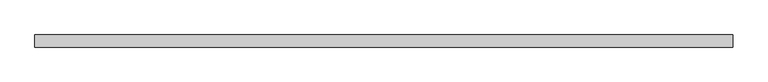
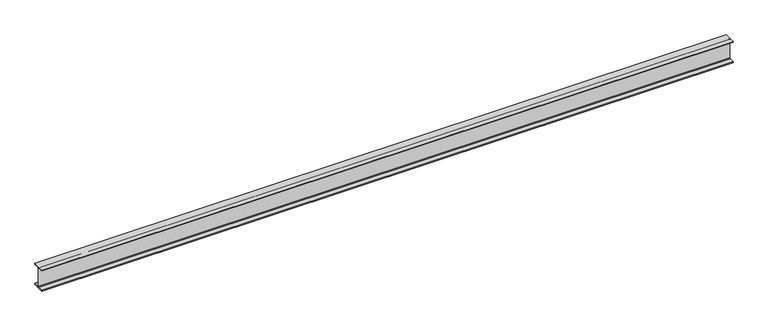
"""IFC4 building model written with IfcOpenShell, lengths in millimetres: beam geometry, Old_Steel Beam_H-KSD3502 : H_SB_ASB_H-350×175x7x11."""

from ifc_helpers import new_model, si_unit, point, frame, frame_2d, origin, place, context, project, spatial, polyline, circle_curve, trimmed, segment, composite_curve, outline, extrude, source, transform, mapped, element, save


def beam_e9001183(model_context):
    return source(origin(), model_context, "Body", "SweptSolid", [
        extrude(outline(composite_curve([segment(polyline([(82.5, -141.5), (82.5, -151.7), (-82.5, -151.7), (-82.5, -141.5), (-11.9, -141.5)]), True, "CONTINUOUS"), segment(trimmed(circle_curve(frame_2d((-11.9, -132.6)), 8.9), [point((-11.9, -141.5))], [point((-3.0, -132.6))], True, "CARTESIAN"), True, "CONTINUOUS"), segment(polyline([(-3.0, -132.6), (-3.0, 132.6)]), True, "CONTINUOUS"), segment(trimmed(circle_curve(frame_2d((-11.9, 132.6)), 8.9), [point((-3.0, 132.6))], [point((-11.9, 141.5))], True, "CARTESIAN"), True, "CONTINUOUS"), segment(polyline([(-11.9, 141.5), (-82.5, 141.5), (-82.5, 151.7), (82.5, 151.7), (82.5, 141.5), (11.9, 141.5)]), True, "CONTINUOUS"), segment(trimmed(circle_curve(frame_2d((11.9, 132.6)), 8.9), [point((11.9, 141.5))], [point((3.0, 132.6))], True, "CARTESIAN"), True, "CONTINUOUS"), segment(polyline([(3.0, 132.6), (3.0, -132.6)]), True, "CONTINUOUS"), segment(trimmed(circle_curve(frame_2d((11.9, -132.6)), 8.9), [point((3.0, -132.6))], [point((11.9, -141.5))], True, "CARTESIAN"), True, "CONTINUOUS"), segment(polyline([(11.9, -141.5), (82.5, -141.5)]), True, "CONTINUOUS")], self_intersect=False)), frame((-4664.4729123, 0.0, 0.0), z_axis=(1.0, 0.0, 0.0), x_axis=(0.0, 1.0, 0.0)), (0.0, 0.0, 1.0), 9526.7729123),
    ])


if __name__ == "__main__":
    model = new_model("IFC4")
    model_context = context("Model", 3, world=origin())
    ifc_project = project(units=[si_unit("LENGTHUNIT", "METRE", prefix="MILLI")], contexts=[model_context])
    site = spatial("IfcSite", under=ifc_project)
    building = spatial("IfcBuilding", under=site)
    placement = place(None, origin())
    beam_shape = beam_e9001183(model_context)
    element("IfcBeam", 1, ObjectType="Old_Steel Beam_H-KSD3502 : H_SB_ASB_H-350×175x7x11", at=placement, inside=building, context=model_context, shape_type="MappedRepresentation", body=[
        mapped(beam_shape, transform((0.0, 0.0, 0.0), x_axis=(1.0, 0.0, 0.0), y_axis=(0.0, 1.0, 0.0), z_axis=(0.0, 0.0, 1.0))),
    ])
    save(model, "model.ifc")

# Revit data of these elements
# Type "Old_Steel Beam_H-KSD3502 : H_SB_ASB_H-350×175x7x11"
#   Width = 17.5 cm
#   Web Thickness = 0.7 cm
#   Web Fillet = 1.4 cm
#   Warping Constant = 282290.0 cm⁶
#   Torsional Moment of Inertia = 19.4042 cm⁴
#   Torsional Modulus = 1.0 cm³
#   Section Area = 63.14 cm²
#   Plastic Modulus weak axis = 174.0 cm³
#   Plastic Modulus strong axis = 868.0 cm³
#   Perimeter = 1.36 m²/m
#   Nominal Weight = 49.60 kgf/m
#   Moment of Inertia weak axis = 984.00 cm⁴
#   Moment of Inertia strong axis = 13600.00 cm⁴
#   Height = 35.0 cm
#   Flange Thickness = 1.1 cm
#   Elastic Modulus weak axis = 112.0 cm³
#   Elastic Modulus strong axis = 775.0 cm³
#   Centroid Vertical = 17.5 cm
#   Centroid Horizontal = 8.75 cm
#   Length [instance default] = 1.5240 m
#   Structural Material [instance default] = Steel, 45-345
#   Assembly Code = ""
# Element 1 (IfcBeam, "Old_Steel Beam_H-KSD3502 : H_SB_ASB_H-350×175x7x11")
#   Structural Material = none
# Materials
#   "Steel, 45-345": class "Metal", colour RGB 189 187 185, transparency 0, Description = "Steel 345 MPa", Cost = 0
